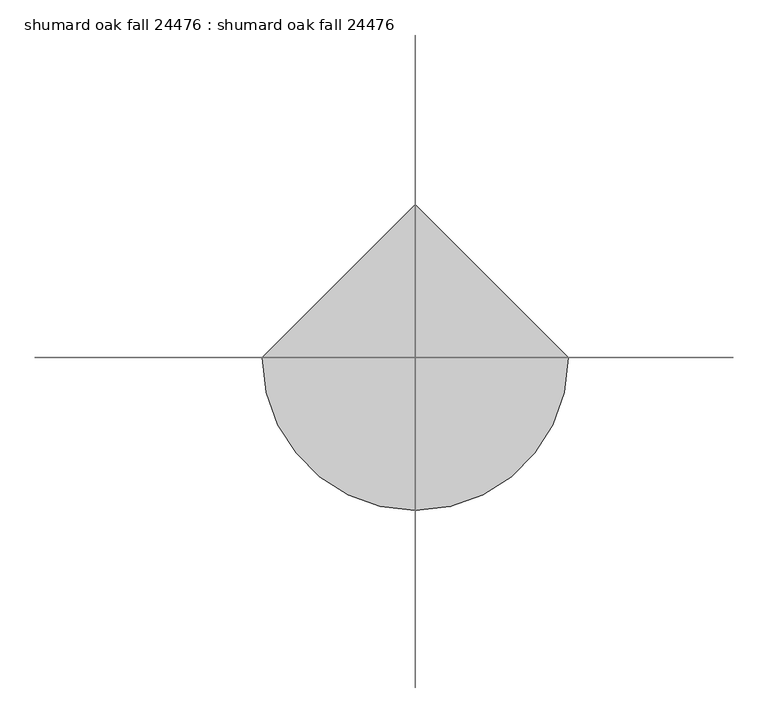
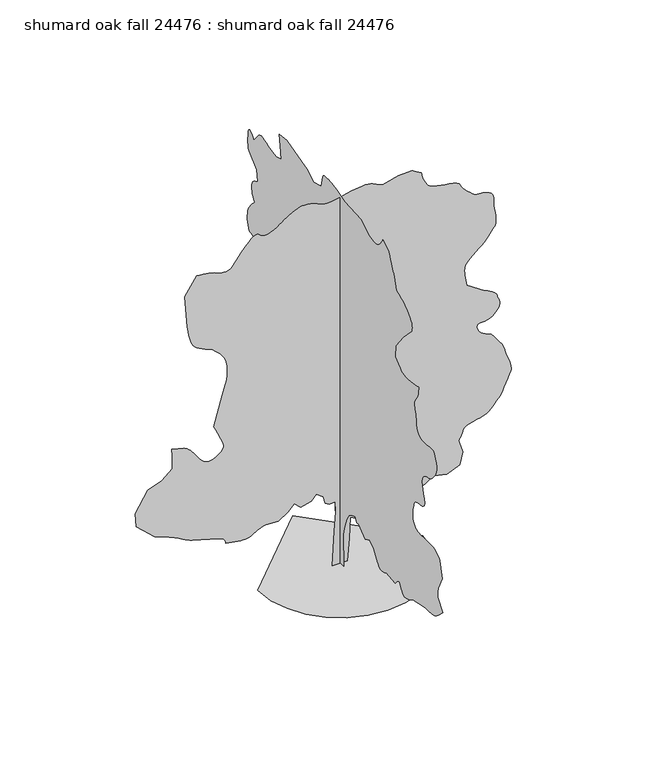
"""IFC4 building model written with IfcOpenShell, lengths in millimetres: proxy geometry, shumard oak fall 24476 : shumard oak fall 24476."""

import ifcopenshell
import ifcopenshell.guid

model = None  # the IFC model being written
_history = None  # IfcOwnerHistory: only IFC2X3 demands one
_inside = {}  # id of a spatial element -> (the spatial element, [elements in it])
_under = {}  # id of a project, library or spatial element -> (it, [spatial elements below it])
_declared = {}  # id of a project -> (the project, [libraries it declares])
_typed = {}  # id of a type object -> (the type object, [elements of that type])
_made_of = {}  # id of a material, layer set ... -> (it, [elements and type objects made of it])


def new_model(schema):
    """Start an empty IFC model of exactly this schema.

    Asked for "IFC4X3", IfcOpenShell would pick the latest addendum, in which some entities
    have other attributes; the version numbers below select the first issue.
    IFC2X3 requires an IfcOwnerHistory on every rooted entity: one is made here for all.
    """
    global model, _history
    if schema == "IFC4X3":
        model = ifcopenshell.file(schema_version=(4, 3, 0, 0))
    else:
        model = ifcopenshell.file(schema=schema)
    _inside.clear()
    _under.clear()
    _declared.clear()
    _typed.clear()
    _made_of.clear()
    _history = None
    if model.schema == "IFC2X3":
        org = make("IfcOrganization", Name="unknown")
        user = make(
            "IfcPersonAndOrganization",
            ThePerson=make("IfcPerson", FamilyName="unknown"),
            TheOrganization=org,
        )
        app = make(
            "IfcApplication",
            ApplicationDeveloper=org,
            Version="unknown",
            ApplicationFullName="unknown",
            ApplicationIdentifier="unknown",
        )
        _history = make(
            "IfcOwnerHistory",
            OwningUser=user,
            OwningApplication=app,
            ChangeAction="ADDED",
            CreationDate=0,
        )
    return model


def make(cls, **values):
    """One entity of the class cls with the attributes given. An attribute that is None is left unset."""
    return model.create_entity(
        cls, **{name: value for name, value in values.items() if value is not None}
    )


def rooted(cls, **values):
    """An entity with a GlobalId (a new one), such as an element, a storey or a relation."""
    return make(cls, GlobalId=ifcopenshell.guid.new(), OwnerHistory=_history, **values)


def si_unit(unit_type, name, prefix=None):
    """IfcSIUnit, for example si_unit("LENGTHUNIT", "METRE", prefix="MILLI")."""
    return make("IfcSIUnit", UnitType=unit_type, Prefix=prefix, Name=name)


def assignment(units):
    """IfcUnitAssignment: the units of a project."""
    return None if units is None else make("IfcUnitAssignment", Units=units)


def point(xyz):
    """IfcCartesianPoint."""
    return None if xyz is None else make("IfcCartesianPoint", Coordinates=xyz)


def direction(xyz):
    """IfcDirection."""
    return None if xyz is None else make("IfcDirection", DirectionRatios=xyz)


def frame(location, z_axis=None, x_axis=None):
    """IfcAxis2Placement3D, a coordinate frame: its origin and axes. An axis left out is left unset."""
    return make(
        "IfcAxis2Placement3D",
        Location=point(location),
        Axis=direction(z_axis),
        RefDirection=direction(x_axis),
    )


def origin():
    """The frame at (0, 0, 0) with its axes left unset."""
    return frame((0.0, 0.0, 0.0))


def place(relative_to, where):
    """IfcLocalPlacement: puts the frame where relative to a parent placement (None: the world)."""
    return make(
        "IfcLocalPlacement", PlacementRelTo=relative_to, RelativePlacement=where
    )


def context(
    kind, dimensions, precision=None, world=None, true_north=None, identifier=None
):
    """IfcGeometricRepresentationContext, for example the 3D "Model" context."""
    return make(
        "IfcGeometricRepresentationContext",
        ContextIdentifier=identifier,
        ContextType=kind,
        CoordinateSpaceDimension=dimensions,
        Precision=precision,
        WorldCoordinateSystem=world,
        TrueNorth=true_north,
    )


def project(units=None, contexts=None):
    """IfcProject with its units and contexts."""
    return rooted(
        "IfcProject",
        Name="project",
        RepresentationContexts=contexts,
        UnitsInContext=assignment(units),
    )


def spatial(cls, under=None, at=None, **own):
    """A site, building, storey or space (cls), placed at a placement, below another one or the project."""
    s = rooted(cls, ObjectPlacement=at, **own)
    if under is not None:
        _under.setdefault(under.id(), (under, []))[1].append(s)
    return s


def point_list(points):
    """IfcCartesianPointList2D or 3D."""
    cls = (
        "IfcCartesianPointList2D" if len(points[0]) == 2 else "IfcCartesianPointList3D"
    )
    return make(cls, CoordList=points)


def triangles(points, corners, closed=None, point_numbers=None):
    """IfcTriangulatedFaceSet: each triangle names its three corners, points numbered from 1."""
    return make(
        "IfcTriangulatedFaceSet",
        Coordinates=point_list(points),
        Closed=closed,
        CoordIndex=corners,
        PnIndex=point_numbers,
    )


def shape(context_of_items, identifier, shape_type, items):
    """IfcShapeRepresentation: the items that make up one representation, for example the "Body"."""
    return make(
        "IfcShapeRepresentation",
        ContextOfItems=context_of_items,
        RepresentationIdentifier=identifier,
        RepresentationType=shape_type,
        Items=items,
    )


def source(mapping_origin, context_of_items, identifier, shape_type, items):
    """IfcRepresentationMap: a shape defined once, which mapped items show again and again."""
    return make(
        "IfcRepresentationMap",
        MappingOrigin=mapping_origin,
        MappedRepresentation=shape(context_of_items, identifier, shape_type, items),
    )


def transform(
    local_origin,
    x_axis=None,
    y_axis=None,
    z_axis=None,
    scale=None,
    scale2=None,
    scale3=None,
    uniform=True,
):
    """IfcCartesianTransformationOperator3D, or its non-uniform kind. x_axis, y_axis, z_axis: its Axis1, 2, 3."""
    if uniform:
        return make(
            "IfcCartesianTransformationOperator3D",
            Axis1=direction(x_axis),
            Axis2=direction(y_axis),
            LocalOrigin=point(local_origin),
            Scale=scale,
            Axis3=direction(z_axis),
        )
    return make(
        "IfcCartesianTransformationOperator3DnonUniform",
        Axis1=direction(x_axis),
        Axis2=direction(y_axis),
        LocalOrigin=point(local_origin),
        Scale=scale,
        Axis3=direction(z_axis),
        Scale2=scale2,
        Scale3=scale3,
    )


def mapped(mapping_source, mapping_target):
    """IfcMappedItem: shows the shape of a source again, moved by a transform."""
    return make(
        "IfcMappedItem", MappingSource=mapping_source, MappingTarget=mapping_target
    )


def made_of(thing, what):
    """Note that an element or type object is made of a material, layer set ...; save() writes the relation."""
    if what is not None:
        _made_of.setdefault(what.id(), (what, []))[1].append(thing)
    return thing


def element(
    cls,
    number,
    at=None,
    inside=None,
    cuts=None,
    type_object=None,
    material=None,
    context=None,
    identifier="Body",
    shape_type=None,
    held_by="IfcProductDefinitionShape",
    body=None,
    shapes=None,
    **own,
):
    """One element of the class cls, such as IfcWall. Its Tag is "e" and its number.

    at: its placement. inside: the storey or other place that contains it. cuts: it is an
    opening in that element (IfcRelVoidsElement). A single representation is given by context,
    identifier, shape_type and body (its items); several are given by shapes. held_by: the class
    of the entity that holds the representations. save() writes the other relations.
    """
    e = rooted(cls, Tag="e%d" % number, ObjectPlacement=at, **own)
    if body is not None:
        shapes = [shape(context, identifier, shape_type, body)]
    if shapes is not None:
        e.Representation = make(held_by, Representations=shapes)
    if inside is not None:
        _inside.setdefault(inside.id(), (inside, []))[1].append(e)
    if cuts is not None:
        rooted(
            "IfcRelVoidsElement", RelatingBuildingElement=cuts, RelatedOpeningElement=e
        )
    if type_object is not None:
        _typed.setdefault(type_object.id(), (type_object, []))[1].append(e)
    return made_of(e, material)


def aggregate(whole, parts):
    """IfcRelAggregates: a whole, such as a stair, and the parts it consists of."""
    return rooted("IfcRelAggregates", RelatingObject=whole, RelatedObjects=parts)


def save(model, path):
    """Write the relations noted so far, then the file.

    IfcRelAggregates (storeys below a building ...), IfcRelContainedInSpatialStructure (elements
    in a storey), IfcRelDefinesByType, IfcRelAssociatesMaterial and IfcRelDeclares: one each for
    every whole, place, type object, material and project.
    """
    for whole, parts in _under.values():
        aggregate(whole, parts)
    for where, things in _inside.values():
        rooted(
            "IfcRelContainedInSpatialStructure",
            RelatedElements=things,
            RelatingStructure=where,
        )
    for kind, things in _typed.values():
        rooted("IfcRelDefinesByType", RelatedObjects=things, RelatingType=kind)
    for what, things in _made_of.values():
        rooted("IfcRelAssociatesMaterial", RelatedObjects=things, RelatingMaterial=what)
    for by, libraries in _declared.values():
        rooted("IfcRelDeclares", RelatingContext=by, RelatedDefinitions=libraries)
    model.write(path)


def shumard_oak_fall_24476_shumard_oak_fall_24476_f3c00e57(model_context):
    return source(origin(), model_context, "Body", "Tessellation", [
        triangles([(-0.002261, 219.4990839, 0.0114695), (-0.002261, -202.1468545, 0.0114695), (-0.002261, -165.4815053, 1044.9594), (-0.002261, -238.8111863, 1356.611816), (-0.002261, -348.8074883, 1649.9305401), (-0.002261, -477.1331583, 1851.5859638), (-0.002261, -623.7925203, 1943.2492641), (-0.002261, -807.1167229, 2016.5789452), (-0.002261, -880.4464039, 1851.5859638), (-0.002261, -1008.7746174, 1888.2507317), (-0.002261, -1155.4339794, 1741.5913696), (-0.002261, -1357.0894032, 1613.2657722), (-0.002261, -1595.4095947, 1723.2602211), (-0.002261, -1815.3986378, 1576.6008591), (-0.002261, -1962.0604706, 1319.9470482), (-0.002261, -1997.5492928, 1269.2765945), (-0.002261, -2033.8382114, 1221.0141335), (-0.002261, -2071.73241, 1177.5624252), (-0.002261, -2112.0319851, 1141.3243029), (-0.002261, -2155.5370331, 1114.7076862), (-0.002261, -2203.0527374, 1100.1179518), (-0.002261, -2255.3767239, 1099.955389), (-0.002261, -2305.5645035, 1108.8834778), (-0.002261, -2347.093364, 1119.7317982), (-0.002261, -2381.4062405, 1132.1853985), (-0.002261, -2409.948103, 1145.9216967), (-0.002261, -2434.1594158, 1160.6206541), (-0.002261, -2455.4852943, 1175.9596888), (-0.002261, -2475.3657669, 1191.618762), (-0.002261, -2952.0087662, 1136.622773), (-0.002261, -2998.9986305, 1190.8694618), (-0.002261, -3044.9978577, 1240.6280525), (-0.002261, -3089.0922592, 1281.4101562), (-0.002261, -3130.3164871, 1308.7227333), (-0.002261, -3167.6796135, 1318.0750694), (-0.002261, -3200.2171623, 1304.9813919), (-0.002261, -3226.9884933, 1264.9485157), (-0.002261, -3253.8871422, 1207.3845148), (-0.002261, -3287.1865631, 1147.8978115), (-0.002261, -3326.5565437, 1091.299086), (-0.002261, -3371.7430298, 1042.3940042), (-0.002261, -3422.3396507, 1005.9958626), (-0.002261, -3478.092643, 986.9154139), (-0.002261, -3538.6462143, 989.9608675), (-0.002261, -3599.3521019, 1007.8145016), (-0.002261, -3656.2224678, 1029.5136858), (-0.002261, -3709.8927383, 1054.4208864), (-0.002261, -3760.9974678, 1081.8909393), (-0.002261, -3810.1717918, 1111.2888542), (-0.002261, -3858.0505554, 1141.9669235), (-0.002261, -3905.294474, 1173.2876135), (-0.002261, -4565.2617485, 1301.6132835), (-0.002261, -4647.5828865, 1301.7733028), (-0.002261, -4728.7613617, 1302.8960541), (-0.002261, -4807.7042175, 1305.9439785), (-0.002261, -4883.2693726, 1311.8748665), (-0.002261, -4954.3638702, 1321.6563915), (-0.002261, -5019.8447571, 1336.2461987), (-0.002261, -5078.5696609, 1356.611816), (-0.002261, -5135.1603928, 1386.0605999), (-0.002261, -5194.6474594, 1426.09086), (-0.002261, -5256.5471695, 1474.9426746), (-0.002261, -5320.3769943, 1530.8479832), (-0.002261, -5385.6294067, 1592.0465733), (-0.002261, -5451.8474579, 1656.7708202), (-0.002261, -5518.5474564, 1723.2602211), (-0.002261, -5261.9061447, 2016.5789452), (-0.002261, -5254.2612625, 2071.5216671), (-0.002261, -5247.8854889, 2126.1442051), (-0.002261, -5244.1008362, 2180.1268112), (-0.002261, -5244.1519958, 2233.1466854), (-0.002261, -5249.3336563, 2284.8837891), (-0.002261, -5260.9410873, 2335.0182289), (-0.002261, -5280.2195618, 2383.2273502), (-0.002261, -5481.8956238, 2804.8665848), (-0.002261, -5353.5493881, 3318.1744972), (-0.002261, -5343.5162796, 3332.34776), (-0.002261, -5313.5698517, 3368.644091), (-0.002261, -5264.0908951, 3417.7422569), (-0.002261, -5195.3584625, 3470.3963104), (-0.002261, -5107.7033478, 3517.2594383), (-0.002261, -5001.4551819, 3549.0601135), (-0.002261, -4876.9191788, 3556.5023918), (-0.002261, -4738.1593346, 3550.7364647), (-0.002261, -4595.2590454, 3548.4758469), (-0.002261, -4457.4642586, 3548.8060593), (-0.002261, -4334.0967888, 3550.7364647), (-0.002261, -4234.4781601, 3553.3020058), (-0.002261, -4167.8793182, 3555.5370438), (-0.002261, -4143.6223686, 3556.5023918), (-0.002261, -4129.3985275, 3566.1797081), (-0.002261, -4092.7461136, 3593.4847275), (-0.002261, -4042.6067322, 3635.877198), (-0.002261, -3987.9714043, 3690.7665802), (-0.002261, -3937.857312, 3755.5873329), (-0.002261, -3901.1798996, 3827.7992043), (-0.002261, -3886.9557678, 3904.8119453), (-0.002261, -3889.6480453, 3981.7738174), (-0.002261, -3897.1159035, 4055.8655159), (-0.002261, -3908.5965981, 4127.5442802), (-0.002261, -3923.3032585, 4197.2923485), (-0.002261, -3940.4225624, 4265.5928307), (-0.002261, -3959.1170609, 4332.9282555), (-0.002261, -3978.6243004, 4399.7808609), (-0.002261, -3994.6515198, 4419.3642586), (-0.002261, -4012.6094353, 4438.4398384), (-0.002261, -4034.4278709, 4456.5497795), (-0.002261, -4062.0122337, 4473.2377144), (-0.002261, -4097.2673492, 4487.969664), (-0.002261, -4142.1744919, 4500.3392578), (-0.002261, -4198.6131981, 4509.7880997), (-0.002261, -4266.863102, 4515.5540268), (-0.002261, -4340.573719, 4522.2850113), (-0.002261, -4411.7190857, 4537.6773857), (-0.002261, -4472.2723663, 4569.4271919), (-0.002261, -4514.2331772, 4625.2310532), (-0.002261, -4529.5493935, 4712.7847206), (-0.002261, -4510.270919, 4839.758947), (-0.002261, -4470.7739113, 4983.3196609), (-0.002261, -4434.4772896, 5115.0185989), (-0.002261, -4406.8420578, 5234.2206253), (-0.002261, -4393.3295105, 5340.2397354), (-0.002261, -4399.3744904, 5432.492244), (-0.002261, -4430.4132935, 5510.3177261), (-0.002261, -4491.9319221, 5573.0557571), (-0.002261, -4567.3444702, 5616.9978424), (-0.002261, -4637.3213036, 5643.9473602), (-0.002261, -4703.1074043, 5661.5747726), (-0.002261, -4766.0230408, 5677.6022827), (-0.002261, -4827.313195, 5699.725351), (-0.002261, -4888.2981354, 5735.6661804), (-0.002261, -4950.2490051, 5793.0446548), (-0.002261, -5013.3678268, 5866.0698486), (-0.002261, -5073.5908951, 5943.8953308), (-0.002261, -5125.8132889, 6026.8263153), (-0.002261, -5164.8783463, 6115.2435928), (-0.002261, -5185.6811462, 6209.4012177), (-0.002261, -5183.0650269, 6309.6799805), (-0.002261, -5151.8989059, 6416.3600967), (-0.002261, -5114.282016, 6517.2737045), (-0.002261, -5088.8312439, 6599.5698441), (-0.002261, -5065.3105865, 6662.6380875), (-0.002261, -5033.4590424, 6705.8180099), (-0.002261, -4983.0150284, 6728.499765), (-0.002261, -4903.6908005, 6729.9985107), (-0.002261, -4785.2506462, 6709.6788208), (-0.002261, -4644.7382927, 6687.2249588), (-0.002261, -4509.6866524, 6682.729303), (-0.002261, -4385.5061508, 6696.2168518), (-0.002261, -4277.7086609, 6727.6364456), (-0.002261, -4191.7298973, 6777.0142456), (-0.002261, -4132.9797043, 6844.3746689), (-0.002261, -4106.9449562, 6929.6677185), (-0.002261, -4098.029512, 7020.7516937), (-0.002261, -4087.1836624, 7106.0447433), (-0.002261, -4074.7123306, 7186.5375046), (-0.002261, -4060.9963074, 7263.169455), (-0.002261, -4046.2896469, 7336.9306503), (-0.002261, -4030.9481415, 7408.761731), (-0.002261, -4015.3017128, 7479.6277542), (-0.002261, -4000.0616547, 7530.732193), (-0.002261, -3987.71735, 7581.9895294), (-0.002261, -3981.1389725, 7633.5764969), (-0.002261, -3983.2216942, 7685.6215759), (-0.002261, -3996.8612686, 7738.3264984), (-0.002261, -4024.9028709, 7791.8185822), (-0.002261, -4070.2925423, 7846.2763046), (-0.002261, -4118.8067322, 7913.1036209), (-0.002261, -4155.4841446, 7996.8979248), (-0.002261, -4181.8746849, 8087.7534256), (-0.002261, -4199.6294151, 8175.7387527), (-0.002261, -4210.3226578, 8250.8719574), (-0.002261, -4215.5551872, 8303.2722473), (-0.002261, -4216.952195, 8322.9315125), (-0.002261, -4189.9012299, 8316.8865326), (-0.002261, -4117.3332756, 8301.5450272), (-0.002261, -4012.0251686, 8281.0724396), (-0.002261, -3886.8543205, 8259.6603745), (-0.002261, -3754.6219849, 8241.4231155), (-0.002261, -3628.1808655, 8230.5772659), (-0.002261, -3520.3075081, 8231.2632706), (-0.002261, -3429.2485313, 8247.1384644), (-0.002261, -3343.9301926, 8277.4401031), (-0.002261, -3263.437722, 8319.7822861), (-0.002261, -3186.8057716, 8371.7250458), (-0.002261, -3113.0442856, 8430.9068985), (-0.002261, -3041.213205, 8494.8640411), (-0.002261, -2970.3474724, 8561.259407), (-0.002261, -2988.6861786, 8946.2469543), (-0.002261, -3391.9868523, 9459.5545761), (-0.002261, -3850.3036446, 9936.1842041), (-0.002261, -3857.4662888, 9995.2898987), (-0.002261, -3860.4634895, 10055.5385468), (-0.002261, -3855.1042236, 10118.0231049), (-0.002261, -3837.2480461, 10183.8597839), (-0.002261, -3802.7295135, 10254.1927002), (-0.002261, -3747.3576027, 10330.1380646), (-0.002261, -3666.9668701, 10412.8399933), (-0.002261, -3572.6822182, 10492.2909576), (-0.002261, -3478.4228554, 10559.2705902), (-0.002261, -3384.1382034, 10615.8113251), (-0.002261, -3289.8535515, 10664.0200104), (-0.002261, -3195.5688995, 10705.9814026), (-0.002261, -3101.2842476, 10743.77677), (-0.002261, -3006.9995956, 10779.4629639), (-0.002261, -2979.491391, 10873.4944336), (-0.002261, -2951.8055809, 10965.8992584), (-0.002261, -2923.7892677, 11055.1042786), (-0.002261, -2895.2904259, 11139.5072662), (-0.002261, -2866.1823189, 11217.4862274), (-0.002261, -2836.2356003, 11287.4366089), (-0.002261, -2805.3494041, 11347.7875763), (-0.002261, -2771.0846352, 11413.5730957), (-0.002261, -2733.3151382, 11494.7518616), (-0.002261, -2695.1895584, 11582.0511841), (-0.002261, -2659.9853119, 11666.1251221), (-0.002261, -2630.8516251, 11737.6765686), (-0.002261, -2611.0141731, 11787.4351593), (-0.002261, -2603.698922, 11806.1037872), (-0.002261, -2292.0441078, 11989.4158539), (-0.002261, -2276.0623798, 11957.8177826), (-0.002261, -2258.4779881, 11925.2813965), (-0.002261, -2237.6856525, 11890.8137329), (-0.002261, -2212.0850349, 11853.4497345), (-0.002261, -2180.0708553, 11812.2255066), (-0.002261, -2140.0379791, 11766.2259888), (-0.002261, -2090.3862133, 11714.4361267), (-0.002261, -2030.5793987, 11669.5795624), (-0.002261, -1962.1138103, 11643.0369965), (-0.002261, -1886.4320927, 11631.6830383), (-0.002261, -1804.9770355, 11632.5469391), (-0.002261, -1719.1937542, 11642.5544678), (-0.002261, -1630.5250385, 11658.6325562), (-0.002261, -1540.413533, 11677.7581329), (-0.002261, -1137.1002874, 11952.7378601), (-0.002261, -257.1441153, 12007.7542694), (-0.002261, -143.4615103, 12039.0221283), (-0.002261, -31.2221381, 12069.3237671), (-0.002261, 78.1307869, 12097.6952911), (-0.002261, 183.1547906, 12123.1972229), (-0.002261, 282.4069083, 12144.8377625), (-0.002261, 374.4436778, 12161.678595), (-0.002261, 457.8190392, 12172.7523376), (-0.002261, 540.0209258, 12181.1855438), (-0.002261, 626.0734131, 12188.6781097), (-0.002261, 710.8406954, 12191.9802338), (-0.002261, 789.1944883, 12187.9165283), (-0.002261, 856.001457, 12173.286026), (-0.002261, 906.1358969, 12144.8377625), (-0.002261, 934.464473, 12099.3975128), (-0.002261, 1026.1253025, 11732.7745422), (-0.002261, 1429.4386208, 11622.7673035), (-0.002261, 1796.0870258, 11842.7562012), (-0.002261, 2254.3987312, 11952.7378601), (-0.002261, 2859.3748856, 12136.0755066), (-0.002261, 3262.6755592, 12081.0846771), (-0.002261, 3226.023436, 11732.7745422), (-0.002261, 3152.6939003, 11329.4491608), (-0.002261, 3446.0126244, 11237.7803375), (-0.002261, 3739.3313484, 11292.771167), (-0.002261, 3852.7421585, 11335.3918213), (-0.002261, 3963.1048988, 11374.2801453), (-0.002261, 4067.3717903, 11405.8258942), (-0.002261, 4162.5200523, 11426.2990631), (-0.002261, 4245.476326, 11432.0138306), (-0.002261, 4313.1925415, 11419.2878632), (-0.002261, 4362.6209198, 11384.4399902), (-0.002261, 4637.600647, 11054.4682709), (-0.002261, 4700.0846237, 11127.5184631), (-0.002261, 4760.3332718, 11191.1203949), (-0.002261, 4816.0609749, 11235.7990631), (-0.002261, 4865.082692, 11252.1062073), (-0.002261, 4905.1133881, 11230.5668243), (-0.002261, 4933.9168625, 11161.7326538), (-0.002261, 4949.2583679, 11036.1298553), (-0.002261, 4953.90634, 10896.6337189), (-0.002261, 4952.7889664, 10788.8868073), (-0.002261, 4946.870723, 10707.5813049), (-0.002261, 4937.0660889, 10647.4593933), (-0.002261, 4924.416861, 10603.2132568), (-0.002261, 4909.8119385, 10569.5327545), (-0.002261, 4894.2675385, 10541.1612305), (-0.002261, 4472.6281586, 10192.8255157), (-0.002261, 4435.9504555, 9807.8641296), (-0.002261, 4494.5989105, 9783.9632629), (-0.002261, 4551.4439873, 9758.1566986), (-0.002261, 4604.7840454, 9728.4893234), (-0.002261, 4652.8407051, 9693.0560211), (-0.002261, 4693.8361679, 9649.9272583), (-0.002261, 4726.0179245, 9597.1711761), (-0.002261, 4747.6078857, 9532.8588226), (-0.002261, 4755.837616, 9462.1706955), (-0.002261, 4750.6050865, 9391.4569885), (-0.002261, 4734.1459167, 9320.7438629), (-0.002261, 4708.6951447, 9250.0301559), (-0.002261, 4676.5133881, 9179.316449), (-0.002261, 4639.8612648, 9108.6033234), (-0.002261, 4600.9485237, 9037.8896164), (-0.002261, 4659.6225586, 8978.9362381), (-0.002261, 4716.8740059, 8919.8305435), (-0.002261, 4771.2299904, 8860.3946365), (-0.002261, 4821.2679245, 8800.4762009), (-0.002261, 4865.5146423, 8739.9229202), (-0.002261, 4902.547847, 8678.581897), (-0.002261, 4930.919371, 8616.2502365), (-0.002261, 4951.2902206, 8555.5446396), (-0.002261, 4965.8951431, 8498.6742737), (-0.002261, 4975.6741974, 8445.0037125), (-0.002261, 4981.5924408, 8393.8992737), (-0.002261, 4984.6405106, 8344.7249496), (-0.002261, 4985.7578842, 8296.8458954), (-0.002261, 4985.9357803, 8249.6022675), (-0.002261, 4875.9285416, 7937.9445465), (-0.002261, 4824.8999702, 7929.765976), (-0.002261, 4773.9984261, 7919.6817078), (-0.002261, 4723.4526741, 7905.7122116), (-0.002261, 4673.363871, 7886.0017868), (-0.002261, 4623.9354927, 7858.5697403), (-0.002261, 4575.2945663, 7821.5365356), (-0.002261, 4527.618988, 7772.9464783), (-0.002261, 4484.2103004, 7715.2883698), (-0.002261, 4447.5581772, 7652.804393), (-0.002261, 4416.4940849, 7586.332869), (-0.002261, 4389.9256485, 7516.635379), (-0.002261, 4366.7354942, 7444.5246643), (-0.002261, 4345.7806686, 7370.8140472), (-0.002261, 4325.9687965, 7296.3162689), (-0.002261, 4283.0426376, 7237.3628906), (-0.002261, 4241.8948586, 7178.257196), (-0.002261, 4204.2520981, 7118.8212891), (-0.002261, 4171.9180252, 7058.9028534), (-0.002261, 4146.6448586, 6998.3489914), (-0.002261, 4130.1856888, 6936.9829697), (-0.002261, 4124.2930252, 6874.676889), (-0.002261, 4142.6317314, 6379.682103), (-0.002261, 4185.5575996, 6375.3643433), (-0.002261, 4226.7056694, 6368.6333588), (-0.002261, 4264.3484299, 6357.076506), (-0.002261, 4296.6825027, 6338.3311386), (-0.002261, 4321.9553787, 6309.9340347), (-0.002261, 4338.4145485, 6269.5481277), (-0.002261, 4344.2819229, 6214.7096146), (-0.002261, 4342.6817299, 6151.3111588), (-0.002261, 4338.2113632, 6086.9732254), (-0.002261, 4331.3027733, 6021.822551), (-0.002261, 4322.4887764, 5956.0108704), (-0.002261, 4312.2271935, 5889.7428223), (-0.002261, 4301.0005531, 5823.1439804), (-0.002261, 4289.2910934, 5756.3928223), (-0.002261, 4270.9523872, 5389.7442719), (-0.002261, 4619.2875206, 5408.0832687), (-0.002261, 5004.2491974, 5481.4130951), (-0.002261, 5086.1895447, 5453.6758347), (-0.002261, 5164.7516098, 5424.4915695), (-0.002261, 5236.6082703, 5392.4115509), (-0.002261, 5298.3300842, 5356.0131912), (-0.002261, 5346.5899292, 5313.8494858), (-0.002261, 5378.009523, 5264.4716858), (-0.002261, 5389.2361633, 5206.4072067), (-0.002261, 5386.0357773, 5132.8744858), (-0.002261, 5377.0444656, 5040.0882889), (-0.002261, 5363.2778641, 4931.2751633), (-0.002261, 5345.6248718, 4809.634623), (-0.002261, 5325.1017059, 4678.3676353), (-0.002261, 5302.6478439, 4540.6745865), (-0.002261, 5279.2545044, 4399.7808609), (-0.002261, 5114.2564362, 3959.8027748), (-0.002261, 5024.1375183, 3909.2570229), (-0.002261, 4935.4661865, 3861.7337608), (-0.002261, 4849.6903175, 3820.3063477), (-0.002261, 4768.2327896, 3788.0228531), (-0.002261, 4692.5661873, 3767.9316376), (-0.002261, 4624.0880997, 3763.0801895), (-0.002261, 4564.2711113, 3776.4912895), (-0.002261, 4050.9631989, 3996.4804779), (-0.002261, 3537.6555771, 3831.4824097), (-0.002261, 3171.0070267, 3574.841098), (-0.002261, 2804.3587669, 3024.8557732), (-0.002261, 2768.8748863, 2970.1951561), (-0.002261, 2732.6038445, 2917.4393646), (-0.002261, 2694.7070297, 2868.5190948), (-0.002261, 2654.3972809, 2825.3897507), (-0.002261, 2610.887146, 2789.9570297), (-0.002261, 2563.3891731, 2764.1504654), (-0.002261, 2511.0525421, 2749.8757553), (-0.002261, 2458.8327644, 2745.1260452), (-0.002261, 2409.8236919, 2745.4815468), (-0.002261, 2360.4918194, 2749.3932266), (-0.002261, 2307.3119259, 2755.2097321), (-0.002261, 2246.7558838, 2761.3564499), (-0.002261, 2175.2957108, 2766.2334778), (-0.002261, 2089.4057499, 2768.2144615), (-0.002261, 1997.2622463, 2761.2550026), (-0.002261, 1908.966909, 2741.798632), (-0.002261, 1823.8796608, 2711.9283623), (-0.002261, 1741.357663, 2673.7013351), (-0.002261, 1660.7585129, 2629.251432), (-0.002261, 1581.4421333, 2580.6105057), (-0.002261, 1502.7683018, 2529.8868576), (-0.002261, 1392.7737076, 2218.2343689), (-0.002261, 1081.123835, 1869.9195831), (-0.002261, 1038.0988449, 1823.313271), (-0.002261, 988.3377834, 1777.6695454), (-0.002261, 932.9658726, 1732.8259163), (-0.002261, 873.1057909, 1688.6248352), (-0.002261, 809.8776735, 1644.9064281), (-0.002261, 744.404199, 1601.5055889), (-0.002261, 677.8105894, 1558.2672398), (-0.002261, 567.8161042, 1943.2492641), (-0.002261, 384.4893582, 2199.9032204), (-0.002261, 311.1621843, 2034.9100937), (-0.002261, 256.16367, 1778.2562828), (-0.002261, 237.8317585, 1319.9470482), (-0.002261, 201.1664093, 678.3109949), (227.1495435, 0.0005814, 0.0290322), (-249.4926201, 0.0005814, 0.0290322), (-176.1637021, 0.0005159, 1099.9731932), (-139.4986073, 0.0004774, 1741.6091011), (-157.8310275, 0.0004578, 2071.5927383), (-341.1570105, 0.0004589, 2053.2615898), (-469.4826805, 0.0004547, 2126.5912708), (-524.4786695, 0.0004403, 2364.9114624), (-744.470256, 0.0004316, 2511.5708244), (-891.1296181, 0.0004414, 2346.5778431), (-1221.1106392, 0.000447, 2254.9170135), (-1422.7685337, 0.0004361, 2438.2411434), (-1624.4239574, 0.000448, 2236.5832489), (-1917.7426815, 0.0004589, 2053.2615898), (-2357.7232384, 0.0004578, 2071.5927383), (-2577.7147522, 0.0004634, 1979.929438), (-2624.9586708, 0.0004655, 1944.816465), (-2672.8377251, 0.0004676, 1911.143811), (-2722.0120491, 0.0004694, 1880.3590622), (-2773.1167786, 0.0004708, 1853.9023922), (-2826.7867584, 0.0004722, 1833.219207), (-2883.6321259, 0.0004729, 1819.7496803), (-2944.3633026, 0.0004732, 1814.9389275), (-3012.0286491, 0.0004732, 1817.0776051), (-3088.3556763, 0.0004729, 1823.0618328), (-3171.8962166, 0.0004722, 1832.2566204), (-3261.2023933, 0.0004715, 1844.0141876), (-3354.8266205, 0.0004708, 1857.6972187), (-3451.3718903, 0.0004697, 1872.662875), (-3549.3394569, 0.000469, 1888.2686085), (-3553.8606926, 0.0004666, 1927.4454323), (-3562.115712, 0.0004641, 1965.9797081), (-3577.7112717, 0.000462, 2003.2338295), (-3604.3811554, 0.0004599, 2038.5626324), (-3645.8085686, 0.0004578, 2071.3260395), (-3705.6508461, 0.0004561, 2100.8815029), (-3787.6420624, 0.0004547, 2126.5912708), (-4594.2684082, 0.0004403, 2364.9114624), (-4660.1306671, 0.0004393, 2385.8106228), (-4730.463002, 0.0004375, 2415.3659409), (-4803.0306656, 0.0004354, 2451.0149277), (-4875.623909, 0.000433, 2490.1916061), (-4945.9562439, 0.0004305, 2530.3313072), (-5011.8185028, 0.0004284, 2568.8757568), (-5070.9241974, 0.0004263, 2603.2419731), (-5134.4749695, 0.0004242, 2636.2617599), (-5213.4178253, 0.0004221, 2672.1773003), (-5305.1878052, 0.0004197, 2710.5057747), (-5407.219368, 0.0004176, 2750.7393654), (-5516.947554, 0.0004151, 2792.446122), (-5631.8062408, 0.0004123, 2835.0926468), (-5749.2298874, 0.0004099, 2878.2217003), (-6317.52892, 0.000378, 3409.8683189), (-6354.1807526, 0.0003518, 3849.846405), (-5969.2187851, 0.0003147, 4473.1359764), (-5529.2409897, 0.0003049, 4638.1340446), (-5199.2448532, 0.0002884, 4913.1140625), (-5199.2448532, 0.0002636, 5334.7534424), (-5217.5832687, 0.0002503, 5554.7423401), (-4832.5963028, 0.0002559, 5463.099678), (-4789.264064, 0.0002576, 5435.1339432), (-4745.0935043, 0.0002594, 5404.4509323), (-4699.3480408, 0.0002615, 5368.3322067), (-4651.1896431, 0.0002639, 5324.0093307), (-4599.8311501, 0.0002674, 5268.8150253), (-4544.4592392, 0.0002716, 5199.9814362), (-4484.2867493, 0.0002765, 5114.7645447), (-4423.3012276, 0.0002818, 5025.254892), (-4364.5513252, 0.0002867, 4946.3120361), (-4305.8264214, 0.0002905, 4879.560878), (-4244.8411903, 0.0002937, 4826.5766121), (-4179.3600128, 0.0002961, 4789.0100098), (-4107.1481415, 0.0002972, 4768.4359749), (-4025.9696663, 0.0002972, 4766.4547005), (-3937.1968872, 0.0002961, 4786.7746811), (-3847.7889725, 0.0002937, 4827.9227509), (-3763.8167725, 0.0002902, 4883.8280594), (-3691.4014252, 0.0002863, 4948.3944672), (-3636.613781, 0.0002825, 5015.5269974), (-3605.5496887, 0.0002786, 5079.1283478), (-3604.3305771, 0.0002755, 5133.1029602), (-3625.9205383, 0.000272, 5191.4720718), (-3658.1020042, 0.0002674, 5270.034137), (-3699.0977577, 0.0002615, 5365.4364532), (-3747.1291283, 0.0002552, 5474.3263184), (-3800.4688957, 0.0002482, 5593.2998703), (-3857.3395523, 0.0002405, 5719.0038254), (-3915.9880074, 0.0002328, 5848.0610641), (-3659.3214066, 0.0001771, 6783.0336456), (-3624.2186073, 0.0001708, 6888.8498611), (-3590.5383957, 0.0001645, 6993.2440704), (-3559.7536469, 0.0001586, 7094.7419449), (-3533.2866577, 0.0001526, 7191.8970612), (-3512.6111755, 0.0001474, 7283.2856689), (-3499.1492065, 0.0001421, 7367.4613449), (-3494.3233383, 0.0001379, 7443.0009201), (-3495.5677391, 0.0001334, 7516.6859573), (-3499.6826042, 0.0001288, 7594.8928116), (-3507.3280678, 0.0001239, 7675.3344131), (-3519.1389748, 0.000119, 7755.7760147), (-3535.7504608, 0.0001145, 7833.9572891), (-3557.8232414, 0.0001099, 7907.6679062), (-3585.9915802, 0.0001061, 7974.6219589), (-3622.2373329, 0.0001022, 8036.9536194), (-3667.1191864, 9.87e-05, 8098.3196411), (-3719.2398422, 9.52e-05, 8158.8735031), (-3777.1264252, 9.14e-05, 8218.7919388), (-3839.3307678, 8.79e-05, 8278.2022659), (-3904.430864, 8.44e-05, 8337.3335403), (-3970.9788368, 8.09e-05, 8396.2869186), (-4076.5918671, 7.84e-05, 8439.5685791), (-4179.4617508, 7.56e-05, 8483.3321869), (-4276.8959198, 7.32e-05, 8528.0870132), (-4366.1768074, 7.04e-05, 8574.2644272), (-4444.5103981, 6.76e-05, 8622.3719559), (-4509.254702, 6.44e-05, 8672.8671295), (-4557.6162849, 6.13e-05, 8726.2574753), (-4595.665416, 5.71e-05, 8797.4537109), (-4630.8443733, 5.15e-05, 8893.9734009), (-4662.4674431, 4.48e-05, 9005.2509109), (-4689.9500679, 3.78e-05, 9120.6938644), (-4712.6068245, 3.12e-05, 9229.7354645), (-4729.828157, 2.59e-05, 9321.7594986), (-4740.9277702, 2.21e-05, 9386.2247498), (-4814.2575966, -3.92e-05, 10412.8399933), (-4447.6090462, -7.32e-05, 10981.1390259), (-4349.6414795, -7.25e-05, 10969.2269623), (-4253.1214989, -7.18e-05, 10956.5009949), (-4159.4719826, -7.07e-05, 10942.1751251), (-4070.1658058, -6.97e-05, 10925.4621918), (-3986.6252655, -6.86e-05, 10905.5238739), (-3910.3238182, -6.72e-05, 10881.5706848), (-3842.658181, -6.55e-05, 10852.8189514), (-3773.849881, -6.37e-05, 10825.0311127), (-3696.4051895, -6.27e-05, 10805.5741608), (-3615.1255577, -6.2e-05, 10796.0491608), (-3534.7854034, -6.23e-05, 10798.0815948), (-3460.2364655, -6.3e-05, 10813.2702026), (-3396.2540337, -6.48e-05, 10843.1916321), (-3347.6639763, -6.76e-05, 10889.4957825), (-3054.3452522, -9.07e-05, 11274.4583313), (-2976.0116615, -9.59e-05, 11364.1447174), (-2898.9227623, -0.0001012, 11449.8185577), (-2824.4246933, -0.0001057, 11527.4917236), (-2753.7618553, -0.0001096, 11593.1260895), (-2688.2300995, -0.0001127, 11642.7312012), (-2629.1244049, -0.0001145, 11672.2724213), (-2577.7147522, -0.0001148, 11677.7837128), (-2536.3434402, -0.0001138, 11663.9915314), (-2502.6707863, -0.0001124, 11641.5382507), (-2470.9233055, -0.000111, 11615.2491577), (-2435.3278038, -0.0001096, 11589.9251221), (-2390.1107964, -0.0001082, 11570.3414337), (-2329.5038853, -0.0001078, 11561.3757019), (-2247.7287895, -0.0001082, 11567.776474), (-2150.0253056, -0.0001099, 11595.5898926), (-2049.7588966, -0.0001124, 11641.9696198), (-1953.3381832, -0.0001159, 11698.6370911), (-1867.1815235, -0.0001194, 11757.2090973), (-1797.6998634, -0.0001225, 11809.3803314), (-1751.3093811, -0.0001246, 11846.7699097), (-1734.4184063, -0.0001257, 11861.0957794), (-1713.7352211, -0.0001264, 11874.3542725), (-1658.7366886, -0.0001285, 11908.7707764), (-1580.0095173, -0.0001313, 11956.3446167), (-1488.1328579, -0.0001344, 12009.0495392), (-1393.6932735, -0.0001372, 12058.8592896), (-1307.269915, -0.0001397, 12097.7720306), (-1239.4444038, -0.0001407, 12117.7615082), (-1175.0935352, -0.0001411, 12122.2065857), (-1095.0303263, -0.0001411, 12119.5648865), (-1003.7428751, -0.0001404, 12109.5829376), (-905.7193525, -0.0001393, 12091.8793671), (-805.4530163, -0.0001379, 12066.1739594), (-707.4294937, -0.0001358, 12032.1388275), (-616.1420425, -0.0001334, 11989.4414337), (-519.0278395, -0.0001313, 11954.5923981), (-402.6731684, -0.0001306, 11941.8675934), (-270.2835022, -0.0001306, 11947.5823608), (-125.0678747, -0.000132, 11968.0543671), (29.7687521, -0.0001337, 11999.5756989), (191.019118, -0.0001362, 12038.4884399), (355.4775026, -0.0001386, 12081.0846771), (468.9975357, -0.0001397, 12096.4767609), (580.1147358, -0.0001404, 12109.9643097), (686.421183, -0.0001411, 12119.5648865), (785.5140444, -0.0001411, 12123.4262787), (874.9828566, -0.0001411, 12119.5648865), (952.4298735, -0.00014, 12106.1029175), (1015.4446318, -0.0001386, 12081.0846771), (1068.3019432, -0.0001369, 12051.7980927), (1117.3137045, -0.0001355, 12026.3729004), (1163.1174494, -0.0001341, 12004.121933), (1206.358342, -0.000133, 11984.4626678), (1247.6713726, -0.000132, 11966.7079376), (1287.7042488, -0.0001309, 11950.2496399), (1327.094577, -0.0001299, 11934.4250244), (1803.737431, -0.0001376, 12062.7706787), (2225.3843685, -0.0001386, 12081.0846771), (2518.7032379, -0.0001288, 11916.111026), (2522.9244919, -0.0001264, 11872.7032104), (2528.9113358, -0.0001236, 11828.1768585), (2538.4235458, -0.0001208, 11781.4157593), (2553.2293282, -0.000118, 11731.2757965), (2575.0986328, -0.0001145, 11676.6663391), (2605.7563545, -0.000111, 11616.417691), (2647.0314514, -0.0001071, 11549.4636383), (2688.5094429, -0.0001033, 11488.1476135), (2722.9265282, -0.0001008, 11442.88526), (2756.7084778, -9.87e-05, 11409.4838104), (2796.2560638, -9.7e-05, 11383.7795654), (2847.995929, -9.59e-05, 11361.5797577), (2918.3282639, -9.45e-05, 11338.7706848), (3013.6797112, -9.28e-05, 11311.1351624), (3131.2053864, -9.14e-05, 11284.5158569), (3258.0272964, -9e-05, 11264.3229034), (3385.509922, -8.89e-05, 11245.7054352), (3504.965712, -8.75e-05, 11223.9114166), (3607.7341484, -8.58e-05, 11194.0923065), (3685.1785492, -8.33e-05, 11151.4204926), (3728.6378151, -7.98e-05, 11091.1462646), (3760.7687027, -7.56e-05, 11020.9656647), (3808.2919647, -7.14e-05, 10951.7512848), (3868.6170616, -6.72e-05, 10883.349646), (3939.2290306, -6.34e-05, 10815.5572723), (4017.5370415, -5.92e-05, 10748.2718445), (4100.9505547, -5.53e-05, 10681.3177917), (4186.9546074, -5.11e-05, 10614.4904755), (4307.9094337, -5.04e-05, 10602.0958832), (4423.8854942, -4.97e-05, 10586.0177948), (4529.9304749, -4.83e-05, 10562.5471344), (4621.0400299, -4.62e-05, 10528.0294739), (4692.2868439, -4.31e-05, 10478.7534119), (4738.6927322, -3.92e-05, 10411.036615), (4755.2533493, -3.4e-05, 10321.1723328), (4756.3201447, -2.84e-05, 10227.5989746), (4759.3173454, -2.35e-05, 10149.3921204), (4763.9147392, -1.96e-05, 10084.03797), (4769.8076935, -1.65e-05, 10028.9448212), (4776.6401253, -1.37e-05, 9981.5232971), (4784.1076927, -1.09e-05, 9939.2584351), (4791.9310524, -8.8e-06, 9899.5329529), (4807.2725578, -3.2e-06, 9805.5782227), (4820.3534454, 2.5e-06, 9713.5286087), (4828.9639664, 7.7e-06, 9625.3398056), (4830.8437935, 1.26e-05, 9542.9425095), (4823.7317276, 1.72e-05, 9468.2156754), (4805.3930214, 2.1e-05, 9403.1155792), (4773.5920555, 2.42e-05, 9349.5729172), (4733.0285431, 2.73e-05, 9298.2138428), (4689.2387741, 3.08e-05, 9239.4639404), (4641.3091415, 3.47e-05, 9174.948111), (4588.2231377, 3.85e-05, 9106.2662567), (4529.0668648, 4.27e-05, 9035.0194427), (4462.8491043, 4.73e-05, 8962.8075714), (4388.6050896, 5.15e-05, 8891.2555435), (4302.3975609, 5.6e-05, 8817.4437698), (4206.2586617, 6.06e-05, 8738.5003326), (4108.1640678, 6.55e-05, 8656.0268784), (4016.1909027, 7.04e-05, 8571.6483078), (3938.3145515, 7.56e-05, 8486.913945), (3882.5615593, 8.05e-05, 8403.5004318), (3856.9584709, 8.54e-05, 8322.9570923), (3852.8436058, 9e-05, 8243.302652), (3855.485305, 9.49e-05, 8161.7436768), (3863.7147446, 9.98e-05, 8078.5842178), (3876.4148415, 0.000105, 7994.1294891), (3892.5185097, 0.0001099, 7908.7347015), (3910.831636, 0.0001152, 7822.6794891), (3930.2880066, 0.0001204, 7736.3196442), (4480.2733315, 0.0001421, 7369.6710938), (4501.5839493, 0.0001428, 7360.1460938), (4556.6003586, 0.0001442, 7333.9587387), (4631.7841415, 0.0001467, 7294.6140472), (4713.7244888, 0.0001495, 7245.668779), (4788.9338516, 0.000153, 7190.60121), (4843.9246811, 0.0001561, 7132.9942612), (4865.2605881, 0.0001596, 7076.3523697), (4876.6907043, 0.0001628, 7022.8347061), (4902.8780594, 0.0001659, 6969.3426224), (4931.6309555, 0.0001694, 6911.3543015), (4950.7571136, 0.0001736, 6844.3746689), (4948.0898346, 0.0001782, 6763.9330673), (4911.438002, 0.0001841, 6665.5588394), (4828.5831757, 0.0001915, 6544.705751), (4714.3087555, 0.0001974, 6441.8614471), (4596.8339493, 0.0002006, 6388.7501541), (4484.1850113, 0.000202, 6367.6938812), (4384.3379082, 0.0002023, 6361.0640533), (4305.3438927, 0.000203, 6351.2344208), (4255.2045113, 0.0002048, 6320.5514099), (4241.9457275, 0.000209, 6251.387027), (4261.0210167, 0.0002139, 6165.12892), (4300.3148392, 0.0002181, 6093.2978394), (4356.423333, 0.0002219, 6033.4811417), (4426.0190849, 0.0002247, 5983.2906006), (4505.7241035, 0.0002272, 5940.3141541), (4592.1348175, 0.0002296, 5902.1629944), (4681.9238136, 0.0002317, 5866.400061), (4771.6616501, 0.0002384, 5752.8878036), (4857.7168625, 0.000245, 5641.7626099), (4936.3806656, 0.0002513, 5535.4638657), (5003.9951431, 0.0002573, 5436.3786346), (5056.8523819, 0.0002629, 5346.8945618), (5091.2694672, 0.0002674, 5269.4504517), (5103.5629028, 0.0002709, 5206.4327866), (5118.5491974, 0.0002755, 5131.0711075), (5155.9631927, 0.0002821, 5023.3247772), (5204.57883, 0.0002895, 4895.6895447), (5253.2194656, 0.0002975, 4760.689064), (5290.633461, 0.0003052, 4630.8190842), (5305.5941757, 0.0003122, 4518.5765167), (5286.899968, 0.0003171, 4436.4838531), (5243.4404114, 0.0003217, 4355.4071159), (5192.9452377, 0.0003283, 4245.7809586), (5137.2939835, 0.000336, 4119.4668663), (5078.4423431, 0.0003437, 3988.3777748), (5018.3210129, 0.0003511, 3864.3243004), (4958.8339462, 0.0003574, 3759.1940895), (4901.913002, 0.0003619, 3684.8483368), (4846.7186966, 0.0003654, 3625.9458275), (4790.2038322, 0.0003693, 3561.6076035), (4731.148716, 0.0003731, 3495.3136848), (4668.2586594, 0.000377, 3430.6455391), (4600.2119408, 0.0003805, 3371.1078941), (4525.7647408, 0.0003836, 3320.2319298), (4443.595919, 0.0003857, 3281.522374), (4346.4919624, 0.0003875, 3252.8203468), (4234.6304764, 0.0003892, 3227.0140732), (4117.9431221, 0.0003906, 3200.2424515), (4006.4118484, 0.0003924, 3168.6449615), (3909.9427368, 0.0003948, 3128.4113708), (3838.4671577, 0.000398, 3075.6555794), (3801.9676414, 0.0004022, 3006.5423561), (3782.4095329, 0.0004064, 2937.2768166), (3757.7209236, 0.0004095, 2883.4033607), (3731.7367538, 0.000412, 2840.121991), (3708.3431236, 0.0004144, 2802.5806778), (3691.325267, 0.0004165, 2766.0302925), (3684.5942825, 0.000419, 2725.6188057), (3691.9856918, 0.0004218, 2676.5715088), (3801.9676414, 0.0004428, 2328.2466946), (3710.2991089, 0.0004666, 1924.9333763), (3306.9984352, 0.0004764, 1759.9428658), (2903.6724724, 0.0004711, 1851.6036953), (2500.3694733, 0.0004862, 1594.9497391), (2207.0507492, 0.0004764, 1759.9428658), (1785.4038116, 0.0004655, 1943.2645248), (1757.7736668, 0.0004666, 1927.1787334), (1729.3384838, 0.0004676, 1908.8451141), (1699.3004917, 0.000469, 1886.0232513), (1666.859594, 0.0004708, 1856.4677879), (1631.2082817, 0.0004729, 1817.9310413), (1591.5512547, 0.000476, 1768.1724506), (1547.0836201, 0.0004799, 1704.9443333), (1500.4771626, 0.0004837, 1638.5081268), (1454.833437, 0.0004872, 1579.7707237), (1409.992424, 0.0004904, 1527.4468826), (1365.7913429, 0.0004932, 1480.2512169), (1322.0704651, 0.0004956, 1436.9061882), (1278.6720966, 0.0004981, 1396.1265553), (1235.4337475, 0.0005005, 1356.6295475), (1290.4296638, 0.0005236, 971.6475231), (1258.8423477, 0.0005243, 960.0499025), (1226.2922997, 0.0005247, 949.5724171), (1191.8194038, 0.0005254, 941.3428322), (1154.4611464, 0.0005257, 936.4787395), (1113.2522518, 0.0005257, 936.1053612), (1067.2326044, 0.0005254, 941.3428322), (1015.4446318, 0.0005247, 953.3138311), (961.5154381, 0.0005233, 973.3035994), (909.5115629, 0.0005219, 1000.9895548), (859.1104242, 0.0005198, 1035.0889996), (809.9919834, 0.0005173, 1074.3192358), (761.8362019, 0.0005149, 1117.3975657), (714.323041, 0.0005121, 1163.0412912), (667.1273752, 0.0005093, 1209.9677147), (318.8101187, 0.0004984, 1393.2944607), (282.1478216, 0.0005387, 714.9936396), (-2555.6678421, 0.0, 0.0), (-2488.1062683, -585.5910004, 0.0), (-2295.6864727, -1123.3614458, 0.0), (-1993.815509, -1597.90639, 0.0), (-1597.90639, -1993.815509, 0.0), (-1123.3614458, -2295.6838566, 0.0), (-585.5910004, -2488.1062683, 0.0), (0.0001117, -2555.6678421, 0.0), (585.5910004, -2488.1062683, 0.0), (1123.3614458, -2295.6864727, 0.0), (1597.90639, -1993.815509, 0.0), (1993.815509, -1597.90639, 0.0), (2295.6864727, -1123.3614458, 0.0), (2488.1062683, -585.5910004, 0.0), (2555.6678421, 0.0002233, 0.0), (-0.0003351, 2555.6678421, 0.0)], [[407, 408, 409], [173, 174, 175], [406, 407, 409], [219, 220, 221], [1, 2, 3], [414, 1, 3], [413, 414, 3], [413, 3, 4], [412, 413, 4], [412, 4, 5], [255, 256, 257], [219, 221, 222], [65, 66, 67], [405, 406, 409], [8, 9, 10], [219, 222, 223], [404, 405, 409], [64, 65, 67], [412, 5, 6], [411, 412, 6], [403, 404, 409], [219, 223, 224], [172, 173, 175], [172, 175, 176], [171, 172, 176], [171, 176, 177], [170, 171, 177], [254, 255, 257], [254, 257, 258], [402, 403, 409], [63, 64, 67], [218, 219, 224], [401, 402, 409], [218, 224, 225], [217, 218, 225], [312, 313, 314], [216, 217, 225], [216, 225, 226], [170, 177, 178], [169, 170, 178], [168, 169, 178], [167, 168, 178], [167, 178, 179], [166, 167, 179], [166, 179, 180], [165, 166, 180], [11, 12, 13], [216, 226, 227], [215, 216, 227], [400, 401, 409], [400, 409, 410], [399, 400, 410], [29, 30, 31], [62, 63, 67], [214, 215, 227], [214, 227, 228], [410, 411, 6], [410, 6, 7], [165, 180, 181], [164, 165, 181], [312, 314, 315], [61, 62, 67], [213, 214, 228], [60, 61, 67], [59, 60, 67], [58, 59, 67], [57, 58, 67], [56, 57, 67], [55, 56, 67], [54, 55, 67], [53, 54, 67], [52, 53, 67], [52, 67, 68], [52, 68, 69], [253, 254, 258], [252, 253, 258], [29, 31, 32], [271, 272, 273], [271, 273, 274], [270, 271, 274], [270, 274, 275], [269, 270, 275], [268, 269, 275], [268, 275, 276], [268, 276, 277], [268, 277, 278], [268, 278, 279], [268, 279, 280], [268, 280, 281], [268, 281, 282], [268, 282, 283], [267, 268, 283], [266, 267, 283], [265, 266, 283], [264, 265, 283], [263, 264, 283], [262, 263, 283], [261, 262, 283], [260, 261, 283], [259, 260, 283], [259, 283, 284], [52, 69, 70], [212, 213, 228], [212, 228, 229], [211, 212, 229], [210, 211, 229], [209, 210, 229], [208, 209, 229], [10, 11, 13], [163, 164, 181], [163, 181, 182], [312, 315, 316], [51, 52, 70], [51, 70, 71], [51, 71, 72], [207, 208, 229], [207, 229, 230], [206, 207, 230], [366, 367, 368], [74, 75, 76], [74, 76, 77], [74, 77, 78], [74, 78, 79], [74, 79, 80], [74, 80, 81], [74, 81, 82], [74, 82, 83], [74, 83, 84], [74, 84, 85], [74, 85, 86], [73, 74, 86], [73, 86, 87], [73, 87, 88], [72, 73, 88], [51, 72, 88], [51, 88, 89], [51, 89, 90], [51, 90, 91], [51, 91, 92], [51, 92, 93], [50, 51, 93], [49, 50, 93], [48, 49, 93], [47, 48, 93], [46, 47, 93], [45, 46, 93], [44, 45, 93], [43, 44, 93], [42, 43, 93], [41, 42, 93], [40, 41, 93], [39, 40, 93], [38, 39, 93], [37, 38, 93], [36, 37, 93], [35, 36, 93], [35, 93, 94], [34, 35, 94], [34, 94, 95], [34, 95, 96], [33, 34, 96], [205, 206, 230], [258, 259, 284], [252, 258, 284], [29, 32, 33], [29, 33, 96], [29, 96, 97], [311, 312, 316], [190, 191, 192], [190, 192, 193], [190, 193, 194], [190, 194, 195], [190, 195, 196], [190, 196, 197], [190, 197, 198], [190, 198, 199], [190, 199, 200], [190, 200, 201], [190, 201, 202], [190, 202, 203], [190, 203, 204], [190, 204, 205], [189, 190, 205], [189, 205, 230], [189, 230, 231], [189, 231, 232], [189, 232, 233], [189, 233, 234], [410, 7, 8], [310, 311, 316], [310, 316, 317], [309, 310, 317], [308, 309, 317], [307, 308, 317], [306, 307, 317], [305, 306, 317], [304, 305, 317], [303, 304, 317], [302, 303, 317], [302, 317, 318], [301, 302, 318], [300, 301, 318], [299, 300, 318], [299, 318, 319], [298, 299, 319], [298, 319, 320], [162, 163, 182], [366, 368, 369], [298, 320, 321], [366, 369, 370], [366, 370, 371], [366, 371, 372], [366, 372, 373], [366, 373, 374], [366, 374, 375], [365, 366, 375], [364, 365, 375], [363, 364, 375], [362, 363, 375], [361, 362, 375], [360, 361, 375], [359, 360, 375], [358, 359, 375], [357, 358, 375], [356, 357, 375], [355, 356, 375], [354, 355, 375], [353, 354, 375], [352, 353, 375], [351, 352, 375], [350, 351, 375], [350, 375, 376], [234, 235, 236], [189, 234, 236], [188, 189, 236], [188, 236, 237], [188, 237, 238], [188, 238, 239], [188, 239, 240], [188, 240, 241], [188, 241, 242], [188, 242, 243], [188, 243, 244], [188, 244, 245], [188, 245, 246], [188, 246, 247], [188, 247, 248], [188, 248, 249], [188, 249, 250], [188, 250, 251], [188, 251, 252], [188, 252, 284], [187, 188, 284], [187, 284, 285], [187, 285, 286], [187, 286, 287], [187, 287, 288], [187, 288, 289], [187, 289, 290], [187, 290, 291], [187, 291, 292], [187, 292, 293], [187, 293, 294], [187, 294, 295], [187, 295, 296], [187, 296, 297], [187, 297, 298], [187, 298, 321], [187, 321, 322], [187, 322, 323], [187, 323, 324], [187, 324, 325], [187, 325, 326], [187, 326, 327], [187, 327, 328], [187, 328, 329], [187, 329, 330], [187, 330, 331], [187, 331, 332], [187, 332, 333], [187, 333, 334], [187, 334, 335], [186, 187, 335], [185, 186, 335], [184, 185, 335], [183, 184, 335], [182, 183, 335], [162, 182, 335], [161, 162, 335], [160, 161, 335], [159, 160, 335], [158, 159, 335], [157, 158, 335], [156, 157, 335], [155, 156, 335], [154, 155, 335], [153, 154, 335], [152, 153, 335], [151, 152, 335], [150, 151, 335], [350, 376, 377], [142, 143, 144], [142, 144, 145], [141, 142, 145], [141, 145, 146], [140, 141, 146], [140, 146, 147], [139, 140, 147], [138, 139, 147], [137, 138, 147], [136, 137, 147], [135, 136, 147], [134, 135, 147], [133, 134, 147], [133, 147, 148], [132, 133, 148], [131, 132, 148], [130, 131, 148], [129, 130, 148], [128, 129, 148], [127, 128, 148], [127, 148, 149], [126, 127, 149], [125, 126, 149], [125, 149, 150], [125, 150, 335], [124, 125, 335], [123, 124, 335], [122, 123, 335], [121, 122, 335], [120, 121, 335], [119, 120, 335], [118, 119, 335], [117, 118, 335], [116, 117, 335], [115, 116, 335], [114, 115, 335], [113, 114, 335], [112, 113, 335], [111, 112, 335], [110, 111, 335], [109, 110, 335], [108, 109, 335], [107, 108, 335], [106, 107, 335], [105, 106, 335], [104, 105, 335], [103, 104, 335], [102, 103, 335], [101, 102, 335], [100, 101, 335], [99, 100, 335], [98, 99, 335], [97, 98, 335], [29, 97, 335], [28, 29, 335], [27, 28, 335], [26, 27, 335], [25, 26, 335], [25, 335, 336], [25, 336, 337], [25, 337, 338], [349, 350, 377], [339, 340, 341], [338, 339, 341], [338, 341, 342], [338, 342, 343], [338, 343, 344], [338, 344, 345], [338, 345, 346], [348, 349, 377], [347, 348, 377], [346, 347, 377], [338, 346, 377], [20, 21, 22], [19, 20, 22], [19, 22, 23], [18, 19, 23], [17, 18, 23], [17, 23, 24], [17, 24, 25], [16, 17, 25], [15, 16, 25], [14, 15, 25], [14, 25, 338], [13, 14, 338], [10, 13, 338], [8, 10, 338], [8, 338, 377], [410, 8, 377], [398, 399, 410], [398, 410, 377], [397, 398, 377], [396, 397, 377], [395, 396, 377], [394, 395, 377], [393, 394, 377], [393, 377, 378], [392, 393, 378], [391, 392, 378], [390, 391, 378], [389, 390, 378], [389, 378, 379], [389, 379, 380], [388, 389, 380], [388, 380, 381], [387, 388, 381], [387, 381, 382], [386, 387, 382], [386, 382, 383], [385, 386, 383], [384, 385, 383], [472, 473, 474], [415, 416, 417], [793, 415, 417], [792, 793, 417], [792, 417, 418], [776, 777, 778], [776, 778, 779], [776, 779, 780], [776, 780, 781], [776, 781, 782], [776, 782, 783], [776, 783, 784], [776, 784, 785], [776, 785, 786], [776, 786, 787], [776, 787, 788], [776, 788, 789], [443, 444, 445], [471, 472, 474], [471, 474, 475], [471, 475, 476], [471, 476, 477], [471, 477, 478], [471, 478, 479], [471, 479, 480], [471, 480, 481], [471, 481, 482], [776, 789, 790], [776, 790, 791], [539, 540, 541], [759, 760, 761], [471, 482, 483], [424, 425, 426], [423, 424, 426], [539, 541, 542], [613, 614, 615], [756, 757, 758], [756, 758, 759], [755, 756, 759], [539, 542, 543], [538, 539, 543], [538, 543, 544], [538, 544, 545], [538, 545, 546], [538, 546, 547], [538, 547, 548], [538, 548, 549], [538, 549, 550], [754, 755, 759], [471, 483, 484], [538, 550, 551], [537, 538, 551], [443, 445, 446], [792, 418, 419], [536, 537, 551], [535, 536, 551], [534, 535, 551], [533, 534, 551], [532, 533, 551], [531, 532, 551], [530, 531, 551], [529, 530, 551], [528, 529, 551], [527, 528, 551], [526, 527, 551], [525, 526, 551], [524, 525, 551], [524, 551, 552], [523, 524, 552], [522, 523, 552], [522, 552, 553], [521, 522, 553], [520, 521, 553], [519, 520, 553], [613, 615, 616], [420, 421, 422], [419, 420, 422], [612, 613, 616], [612, 616, 617], [612, 617, 618], [612, 618, 619], [776, 791, 792], [776, 792, 419], [775, 776, 419], [774, 775, 419], [773, 774, 419], [772, 773, 419], [771, 772, 419], [770, 771, 419], [769, 770, 419], [768, 769, 419], [767, 768, 419], [766, 767, 419], [765, 766, 419], [764, 765, 419], [466, 467, 468], [466, 468, 469], [466, 469, 470], [465, 466, 470], [464, 465, 470], [463, 464, 470], [462, 463, 470], [461, 462, 470], [461, 470, 471], [461, 471, 484], [461, 484, 485], [461, 485, 486], [460, 461, 486], [459, 460, 486], [459, 486, 487], [458, 459, 487], [457, 458, 487], [456, 457, 487], [455, 456, 487], [454, 455, 487], [453, 454, 487], [452, 453, 487], [451, 452, 487], [451, 487, 488], [451, 488, 489], [450, 451, 489], [450, 489, 490], [449, 450, 490], [449, 490, 491], [449, 491, 492], [448, 449, 492], [518, 519, 553], [518, 553, 554], [611, 612, 619], [611, 619, 620], [611, 620, 621], [448, 492, 493], [754, 759, 761], [754, 761, 762], [753, 754, 762], [752, 753, 762], [501, 502, 503], [611, 621, 622], [763, 764, 419], [447, 448, 493], [517, 518, 554], [500, 501, 503], [611, 622, 623], [762, 763, 419], [762, 419, 422], [752, 762, 422], [751, 752, 422], [750, 751, 422], [749, 750, 422], [748, 749, 422], [747, 748, 422], [747, 422, 423], [427, 428, 429], [517, 554, 555], [426, 427, 429], [517, 555, 556], [516, 517, 556], [516, 556, 557], [516, 557, 558], [516, 558, 559], [516, 559, 560], [516, 560, 561], [516, 561, 562], [516, 562, 563], [516, 563, 564], [516, 564, 565], [516, 565, 566], [516, 566, 567], [516, 567, 568], [516, 568, 569], [516, 569, 570], [516, 570, 571], [515, 516, 571], [515, 571, 572], [514, 515, 572], [514, 572, 573], [442, 443, 446], [442, 446, 447], [442, 447, 493], [441, 442, 493], [440, 441, 493], [439, 440, 493], [438, 439, 493], [437, 438, 493], [436, 437, 493], [435, 436, 493], [434, 435, 493], [433, 434, 493], [432, 433, 493], [431, 432, 493], [430, 431, 493], [429, 430, 493], [426, 429, 493], [426, 493, 494], [423, 426, 494], [423, 494, 495], [747, 423, 495], [747, 495, 496], [746, 747, 496], [746, 496, 497], [746, 497, 498], [746, 498, 499], [746, 499, 500], [746, 500, 503], [746, 503, 504], [746, 504, 505], [746, 505, 506], [746, 506, 507], [746, 507, 508], [746, 508, 509], [746, 509, 510], [746, 510, 511], [746, 511, 512], [745, 746, 512], [745, 512, 513], [745, 513, 514], [745, 514, 573], [745, 573, 574], [745, 574, 575], [745, 575, 576], [745, 576, 577], [745, 577, 578], [745, 578, 579], [745, 579, 580], [745, 580, 581], [745, 581, 582], [745, 582, 583], [745, 583, 584], [745, 584, 585], [745, 585, 586], [745, 586, 587], [745, 587, 588], [745, 588, 589], [745, 589, 590], [745, 590, 591], [745, 591, 592], [745, 592, 593], [745, 593, 594], [745, 594, 595], [745, 595, 596], [745, 596, 597], [745, 597, 598], [745, 598, 599], [745, 599, 600], [745, 600, 601], [745, 601, 602], [745, 602, 603], [745, 603, 604], [745, 604, 605], [745, 605, 606], [745, 606, 607], [745, 607, 608], [745, 608, 609], [745, 609, 610], [745, 610, 611], [745, 611, 623], [745, 623, 624], [745, 624, 625], [745, 625, 626], [745, 626, 627], [745, 627, 628], [745, 628, 629], [745, 629, 630], [745, 630, 631], [745, 631, 632], [745, 632, 633], [745, 633, 634], [745, 634, 635], [745, 635, 636], [712, 713, 714], [647, 648, 649], [646, 647, 649], [645, 646, 649], [645, 649, 650], [644, 645, 650], [644, 650, 651], [643, 644, 651], [643, 651, 652], [642, 643, 652], [642, 652, 653], [642, 653, 654], [642, 654, 655], [642, 655, 656], [642, 656, 657], [642, 657, 658], [642, 658, 659], [642, 659, 660], [642, 660, 661], [642, 661, 662], [642, 662, 663], [642, 663, 664], [642, 664, 665], [642, 665, 666], [642, 666, 667], [642, 667, 668], [642, 668, 669], [642, 669, 670], [642, 670, 671], [642, 671, 672], [641, 642, 672], [641, 672, 673], [640, 641, 673], [640, 673, 674], [639, 640, 674], [639, 674, 675], [638, 639, 675], [637, 638, 675], [637, 675, 676], [636, 637, 676], [690, 691, 692], [690, 692, 693], [689, 690, 693], [688, 689, 693], [725, 726, 727], [725, 727, 728], [724, 725, 728], [724, 728, 729], [723, 724, 729], [723, 729, 730], [722, 723, 730], [722, 730, 731], [721, 722, 731], [721, 731, 732], [721, 732, 733], [721, 733, 734], [721, 734, 735], [721, 735, 736], [721, 736, 737], [721, 737, 738], [721, 738, 739], [721, 739, 740], [721, 740, 741], [721, 741, 742], [721, 742, 743], [721, 743, 744], [721, 744, 745], [720, 721, 745], [719, 720, 745], [718, 719, 745], [717, 718, 745], [716, 717, 745], [715, 716, 745], [714, 715, 745], [712, 714, 745], [711, 712, 745], [710, 711, 745], [709, 710, 745], [708, 709, 745], [707, 708, 745], [687, 688, 693], [636, 676, 677], [687, 693, 694], [686, 687, 694], [685, 686, 694], [685, 694, 695], [685, 695, 696], [685, 696, 697], [685, 697, 698], [685, 698, 699], [685, 699, 700], [685, 700, 701], [685, 701, 702], [685, 702, 703], [685, 703, 704], [684, 685, 704], [684, 704, 705], [684, 705, 706], [706, 707, 745], [684, 706, 745], [683, 684, 745], [682, 683, 745], [681, 682, 745], [680, 681, 745], [636, 677, 678], [745, 636, 678], [745, 678, 679], [680, 745, 679], [808, 809, 794], [807, 808, 794], [807, 794, 795], [806, 807, 795], [806, 795, 796], [806, 796, 797], [805, 806, 797], [804, 805, 797], [804, 797, 798], [804, 798, 799], [804, 799, 800], [804, 800, 801], [804, 801, 802], [804, 802, 803]], closed=False),
    ])


if __name__ == "__main__":
    model = new_model("IFC4")
    model_context = context("Model", 3, world=origin())
    ifc_project = project(units=[si_unit("LENGTHUNIT", "METRE", prefix="MILLI")], contexts=[model_context])
    site = spatial("IfcSite", under=ifc_project)
    building = spatial("IfcBuilding", under=site)
    placement = place(None, origin())
    shumard_oak_fall_24476_shumard_oak_fall_24476_shape = shumard_oak_fall_24476_shumard_oak_fall_24476_f3c00e57(model_context)
    element("IfcBuildingElementProxy", 1, Name="shumard oak fall 24476 : shumard oak fall 24476", ObjectType="shumard oak fall 24476 : shumard oak fall 24476", at=placement, inside=building, context=model_context, shape_type="MappedRepresentation", body=[
        mapped(shumard_oak_fall_24476_shumard_oak_fall_24476_shape, transform((0.0, 0.0, 0.0), x_axis=(1.0, 0.0, 0.0), y_axis=(0.0, 1.0, 0.0), z_axis=(0.0, 0.0, 1.0))),
    ])
    save(model, "model.ifc")

# Revit data of these elements
# Type "shumard oak fall 24476 : shumard oak fall 24476"
#   built-in parameter 1005195 = "RPC-16-FXGN-6JXX-PG4N-6000-ST1L-LVER-AU"
#   Height = 0
